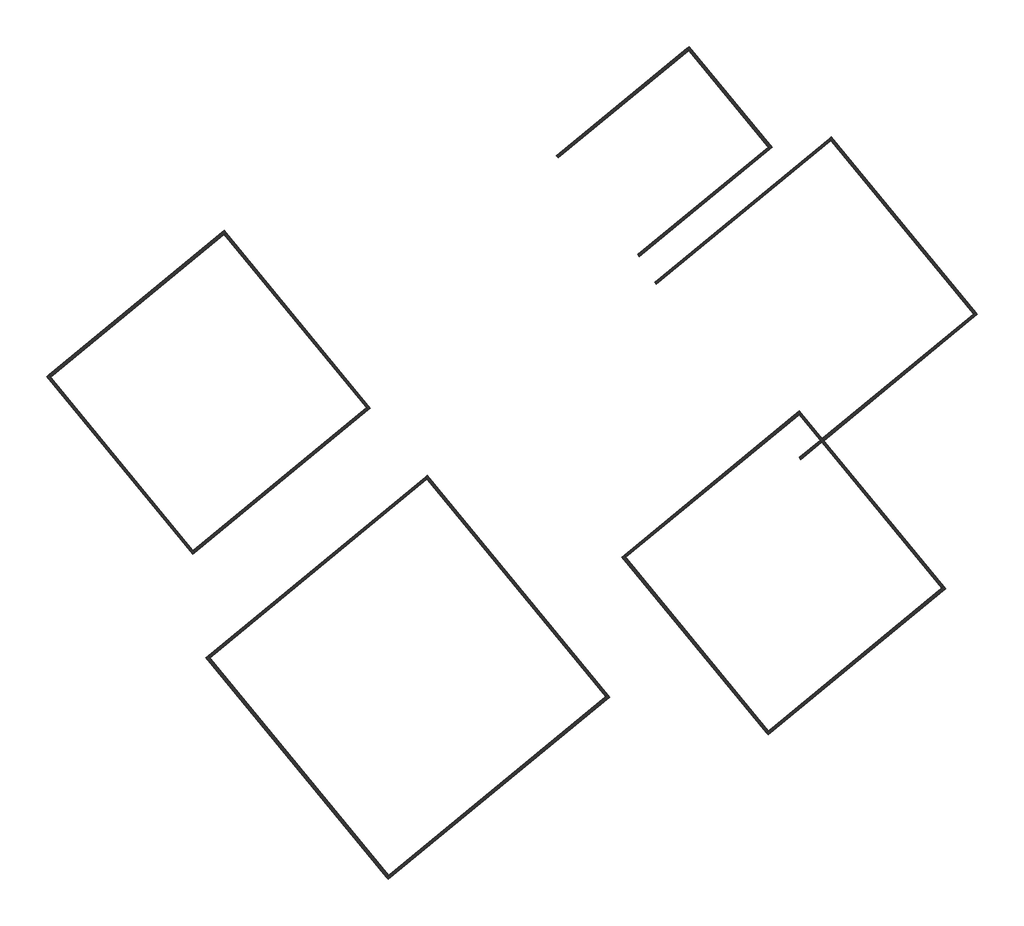
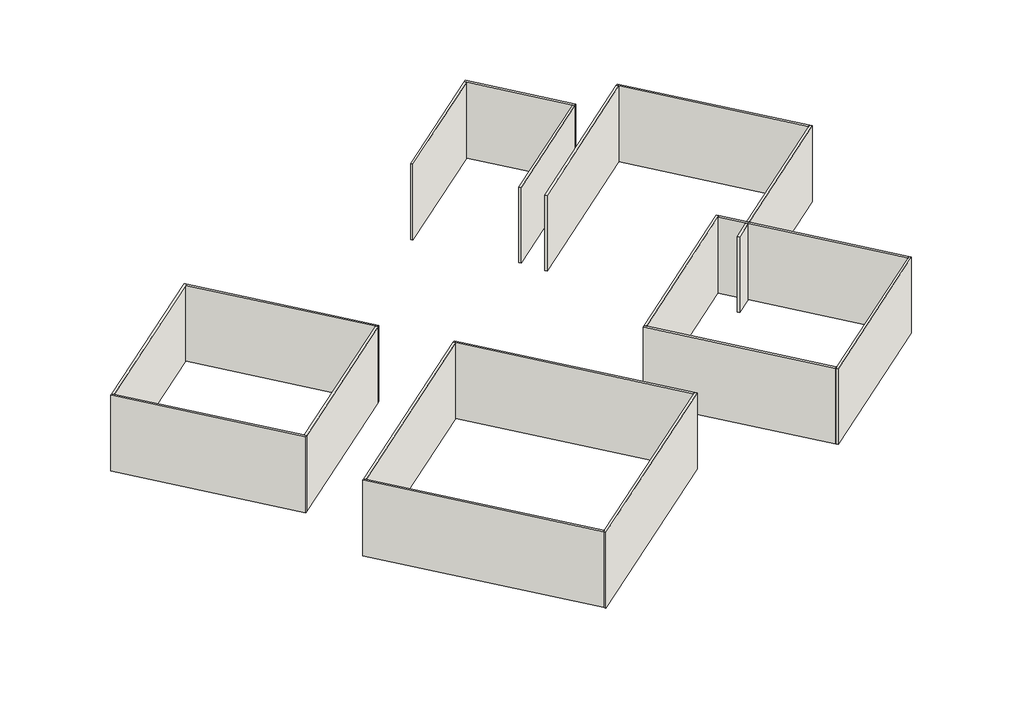
# One storey: 18 walls.
"""IFC4 building model written with IfcOpenShell, lengths in millimetres."""

from ifc_helpers import new_model, si_unit, frame, origin, place, context, project, spatial, polyline, outline, extrude, faceted_brep, element, save

model = new_model("IFC4")

# Units and contexts
model_context = context("Model", 3, world=origin())
ifc_project = project(units=[si_unit("LENGTHUNIT", "METRE", prefix="MILLI")], contexts=[model_context])

# Site, building, storey
site = spatial("IfcSite", under=ifc_project)
building = spatial("IfcBuilding", under=site)
storey = spatial("IfcBuildingStorey", under=building, Name="f3-展厅", Elevation=17500.0)

# Walls
placement = place(None, origin())
element("IfcWall", 1, ObjectType="aa-大理石-米黄色 - 200mm", at=placement, inside=storey, context=model_context, shape_type="Brep", body=[
    faceted_brep([(-29489.0476402, -25007.5608793, 17500.0), (-13891.5005151, -12171.8091024, 17500.0), (-13891.5005151, -12171.8091024, 24700.0), (-29489.0476402, -25007.5608793, 24700.0), (-29616.1342915, -24853.1297197, 17500.0), (-29616.1342915, -24853.1297197, 24700.0), (-29461.7031318, -24726.0430684, 24700.0), (-14173.018326, -12144.464594, 24700.0), (-14018.5871664, -12017.3779427, 24700.0), (-14018.5871664, -12017.3779427, 17500.0), (-14173.018326, -12144.464594, 17500.0), (-29461.7031318, -24726.0430684, 17500.0)], [[[0, 1, 2, 3]], [[4, 5, 6, 7, 8, 9, 10, 11]], [[1, 0, 4, 11, 10, 9]], [[3, 2, 8, 7, 6, 5]], [[2, 1, 9, 8]], [[0, 3, 5, 4]]]),
])
element("IfcWall", 2, ObjectType="aa-大理石-米黄色 - 200mm", at=placement, inside=storey, context=model_context, shape_type="Brep", body=[
    faceted_brep([(-14018.5871664, -12017.3779427, 17500.0), (-26727.2522921, 3425.7380228, 17500.0), (-26727.2522921, 3425.7380228, 24700.0), (-14018.5871664, -12017.3779427, 24700.0), (-14173.018326, -12144.464594, 17500.0), (-14173.018326, -12144.464594, 24700.0), (-26754.5968005, 3144.2202119, 24700.0), (-26881.6834517, 3298.6513715, 24700.0), (-26881.6834517, 3298.6513715, 17500.0), (-26754.5968005, 3144.2202119, 17500.0)], [[[0, 1, 2, 3]], [[4, 5, 6, 7, 8, 9]], [[1, 0, 4, 9, 8]], [[3, 2, 7, 6, 5]], [[0, 3, 5, 4]], [[2, 1, 8, 7]]]),
])
element("IfcWall", 3, ObjectType="aa-大理石-米黄色 - 200mm", at=placement, inside=storey, context=model_context, shape_type="Brep", body=[
    faceted_brep([(-42324.7994172, -9410.0137542, 17500.0), (-29616.1342915, -24853.1297197, 17500.0), (-29616.1342915, -24853.1297197, 24700.0), (-42324.7994172, -9410.0137542, 24700.0), (-42170.3682575, -9282.9271029, 17500.0), (-42170.3682575, -9282.9271029, 24700.0), (-42043.2816063, -9437.3582626, 24700.0), (-29461.7031318, -24726.0430684, 24700.0), (-29461.7031318, -24726.0430684, 17500.0), (-42043.2816063, -9437.3582626, 17500.0)], [[[0, 1, 2, 3]], [[4, 5, 6, 7, 8, 9]], [[1, 0, 4, 9, 8]], [[3, 2, 7, 6, 5]], [[2, 1, 8, 7]], [[0, 3, 5, 4]]]),
])
element("IfcWall", 4, ObjectType="aa-大理石-米黄色 - 200mm", at=placement, inside=storey, context=model_context, shape_type="SweptSolid", body=[
    extrude(outline(polyline([(-42170.3682575, -9282.9271029), (-26881.6834517, 3298.6513715), (-26754.5968005, 3144.2202119), (-42043.2816063, -9437.3582626), (-42170.3682575, -9282.9271029)])), frame((0.0, 0.0, 17500.0), z_axis=(0.0, 0.0, 1.0), x_axis=(1.0, 0.0, 0.0)), (0.0, 0.0, 1.0), 7200.0),
])
element("IfcWall", 5, ObjectType="aa-大理石-米黄色 - 200mm", at=placement, inside=storey, context=model_context, shape_type="Brep", body=[
    faceted_brep([(-53539.2738644, 10380.4187427, 17500.0), (-43245.2551126, -2128.5051893, 17500.0), (-43245.2551126, -2128.5051893, 24700.0), (-53539.2738644, 10380.4187427, 24700.0), (-53384.8427048, 10507.505394, 17500.0), (-53384.8427048, 10507.505394, 24700.0), (-53257.7560535, 10353.0742343, 24700.0), (-43217.9106042, -1846.9873784, 24700.0), (-43090.823953, -2001.418538, 24700.0), (-43090.823953, -2001.418538, 17500.0), (-43217.9106042, -1846.9873784, 17500.0), (-53257.7560535, 10353.0742343, 17500.0)], [[[0, 1, 2, 3]], [[4, 5, 6, 7, 8, 9, 10, 11]], [[1, 0, 4, 11, 10, 9]], [[3, 2, 8, 7, 6, 5]], [[0, 3, 5, 4]], [[2, 1, 9, 8]]]),
])
element("IfcWall", 6, ObjectType="aa-大理石-米黄色 - 200mm", at=placement, inside=storey, context=model_context, shape_type="Brep", body=[
    faceted_brep([(-41030.3499324, 20674.4374946, 17500.0), (-53384.8427048, 10507.505394, 17500.0), (-53384.8427048, 10507.505394, 24700.0), (-41030.3499324, 20674.4374946, 24700.0), (-40903.2632812, 20520.0063349, 17500.0), (-40903.2632812, 20520.0063349, 24700.0), (-41057.6944408, 20392.9196836, 24700.0), (-53257.7560535, 10353.0742343, 24700.0), (-53257.7560535, 10353.0742343, 17500.0), (-41057.6944408, 20392.9196836, 17500.0)], [[[0, 1, 2, 3]], [[4, 5, 6, 7, 8, 9]], [[1, 0, 4, 9, 8]], [[3, 2, 7, 6, 5]], [[2, 1, 8, 7]], [[0, 3, 5, 4]]]),
])
element("IfcWall", 7, ObjectType="aa-大理石-米黄色 - 200mm", at=placement, inside=storey, context=model_context, shape_type="Brep", body=[
    faceted_brep([(-30736.3311806, 8165.5135625, 17500.0), (-40903.2632812, 20520.0063349, 17500.0), (-40903.2632812, 20520.0063349, 24700.0), (-30736.3311806, 8165.5135625, 24700.0), (-30890.7623403, 8038.4269113, 17500.0), (-30890.7623403, 8038.4269113, 24700.0), (-31017.8489915, 8192.8580709, 24700.0), (-41057.6944408, 20392.9196836, 24700.0), (-41057.6944408, 20392.9196836, 17500.0), (-31017.8489915, 8192.8580709, 17500.0)], [[[0, 1, 2, 3]], [[4, 5, 6, 7, 8, 9]], [[1, 0, 4, 9, 8]], [[3, 2, 7, 6, 5]], [[2, 1, 8, 7]], [[0, 3, 5, 4]]]),
])
element("IfcWall", 8, ObjectType="aa-大理石-米黄色 - 200mm", at=placement, inside=storey, context=model_context, shape_type="SweptSolid", body=[
    extrude(outline(polyline([(-30890.7623403, 8038.4269113), (-43090.823953, -2001.418538), (-43217.9106042, -1846.9873784), (-31017.8489915, 8192.8580709), (-30890.7623403, 8038.4269113)])), frame((0.0, 0.0, 17500.0), z_axis=(0.0, 0.0, 1.0), x_axis=(1.0, 0.0, 0.0)), (0.0, 0.0, 1.0), 7200.0),
])
element("IfcWall", 9, ObjectType="aa-大理石-米黄色 - 200mm", at=placement, inside=storey, context=model_context, shape_type="Brep", body=[
    faceted_brep([(-2742.3908548, -14827.0816231, 17500.0), (9766.5330772, -4533.0628713, 17500.0), (9766.5330772, -4533.0628713, 24700.0), (-2742.3908548, -14827.0816231, 24700.0), (-2869.4775061, -14672.6504634, 17500.0), (-2869.4775061, -14672.6504634, 24700.0), (-2715.0463464, -14545.5638122, 24700.0), (9485.0152663, -4505.7183629, 24700.0), (9639.446426, -4378.6317116, 24700.0), (9639.446426, -4378.6317116, 17500.0), (9485.0152663, -4505.7183629, 17500.0), (-2715.0463464, -14545.5638122, 17500.0)], [[[0, 1, 2, 3]], [[4, 5, 6, 7, 8, 9, 10, 11]], [[1, 0, 4, 11, 10, 9]], [[3, 2, 8, 7, 6, 5]], [[0, 3, 5, 4]], [[2, 1, 9, 8]]]),
])
element("IfcWall", 10, ObjectType="aa-大理石-米黄色 - 200mm", at=placement, inside=storey, context=model_context, shape_type="Brep", body=[
    faceted_brep([(-13036.4096066, -2318.157691, 17500.0), (-2869.4775061, -14672.6504634, 17500.0), (-2869.4775061, -14672.6504634, 24700.0), (-13036.4096066, -2318.157691, 24700.0), (-12881.978447, -2191.0710398, 17500.0), (-12881.978447, -2191.0710398, 24700.0), (-12754.8917957, -2345.5021994, 24700.0), (-2715.0463464, -14545.5638122, 24700.0), (-2715.0463464, -14545.5638122, 17500.0), (-12754.8917957, -2345.5021994, 17500.0)], [[[0, 1, 2, 3]], [[4, 5, 6, 7, 8, 9]], [[1, 0, 4, 9, 8]], [[3, 2, 7, 6, 5]], [[2, 1, 8, 7]], [[0, 3, 5, 4]]]),
])
element("IfcWall", 11, ObjectType="aa-大理石-米黄色 - 200mm", at=placement, inside=storey, context=model_context, shape_type="Brep", body=[
    faceted_brep([(-527.4856746, 7975.8610608, 17500.0), (-12881.978447, -2191.0710398, 17500.0), (-12881.978447, -2191.0710398, 24700.0), (-527.4856746, 7975.8610608, 24700.0), (-400.3990233, 7821.4299011, 17500.0), (-400.3990233, 7821.4299011, 24700.0), (-554.830183, 7694.3432499, 24700.0), (-12754.8917957, -2345.5021994, 24700.0), (-12754.8917957, -2345.5021994, 17500.0), (-554.830183, 7694.3432499, 17500.0)], [[[0, 1, 2, 3]], [[4, 5, 6, 7, 8, 9]], [[1, 0, 4, 9, 8]], [[3, 2, 7, 6, 5]], [[2, 1, 8, 7]], [[0, 3, 5, 4]]]),
])
element("IfcWall", 12, ObjectType="aa-大理石-米黄色 - 200mm", at=placement, inside=storey, context=model_context, shape_type="Brep", body=[
    faceted_brep([(9639.446426, -4378.6317116, 17500.0), (1199.9237396, 5876.7748358, 17500.0), (1072.8370883, 6031.2059954, 17500.0), (-400.3990233, 7821.4299011, 17500.0), (-400.3990233, 7821.4299011, 24700.0), (1072.8370883, 6031.2059954, 24700.0), (1199.9237396, 5876.7748358, 24700.0), (9639.446426, -4378.6317116, 24700.0), (9485.0152663, -4505.7183629, 17500.0), (9485.0152663, -4505.7183629, 24700.0), (1045.4925799, 5749.6881845, 24700.0), (918.4059287, 5904.1193442, 24700.0), (-554.830183, 7694.3432499, 24700.0), (-554.830183, 7694.3432499, 17500.0), (918.4059287, 5904.1193442, 17500.0), (1045.4925799, 5749.6881845, 17500.0)], [[[0, 1, 2, 3, 4, 5, 6, 7]], [[8, 9, 10, 11, 12, 13, 14, 15]], [[3, 2, 1, 0, 8, 15, 14, 13]], [[7, 6, 5, 4, 12, 11, 10, 9]], [[0, 7, 9, 8]], [[4, 3, 13, 12]]]),
])
element("IfcWall", 13, ObjectType="aa-大理石-米黄色 - 200mm", at=placement, inside=storey, context=model_context, shape_type="Brep", body=[
    faceted_brep([(-429.0438457, 4536.2420322, 24700.0), (-429.0438457, 4536.2420322, 17500.0), (1045.4925799, 5749.6881845, 17500.0), (1045.4925799, 5749.6881845, 24700.0), (-556.1304969, 4690.6731918, 17500.0), (-556.1304969, 4690.6731918, 24700.0), (918.4059287, 5904.1193442, 24700.0), (918.4059287, 5904.1193442, 17500.0)], [[[0, 1, 2, 3]], [[4, 5, 6, 7]], [[1, 4, 7, 2]], [[5, 0, 3, 6]], [[1, 0, 5, 4]], [[3, 2, 7, 6]]]),
    faceted_brep([(12002.6645065, 14766.7174583, 17500.0), (12002.6645065, 14766.7174583, 24700.0), (1199.9237396, 5876.7748358, 24700.0), (1199.9237396, 5876.7748358, 17500.0), (11875.5778553, 14921.148618, 24700.0), (11875.5778553, 14921.148618, 17500.0), (11721.1466956, 14794.0619667, 17500.0), (1072.8370883, 6031.2059954, 17500.0), (1072.8370883, 6031.2059954, 24700.0), (11721.1466956, 14794.0619667, 24700.0)], [[[0, 1, 2, 3]], [[4, 5, 6, 7, 8, 9]], [[5, 0, 3, 7, 6]], [[1, 4, 9, 8, 2]], [[3, 2, 8, 7]], [[1, 0, 5, 4]]]),
])
element("IfcWall", 14, ObjectType="aa-大理石-米黄色 - 200mm", at=placement, inside=storey, context=model_context, shape_type="Brep", body=[
    faceted_brep([(11875.5778553, 14921.148618, 17500.0), (1708.6457547, 27275.6413904, 17500.0), (1708.6457547, 27275.6413904, 24700.0), (11875.5778553, 14921.148618, 24700.0), (11721.1466956, 14794.0619667, 17500.0), (11721.1466956, 14794.0619667, 24700.0), (1681.3012463, 26994.1235795, 24700.0), (1554.2145951, 27148.5547391, 24700.0), (1554.2145951, 27148.5547391, 17500.0), (1681.3012463, 26994.1235795, 17500.0)], [[[0, 1, 2, 3]], [[4, 5, 6, 7, 8, 9]], [[1, 0, 4, 9, 8]], [[3, 2, 7, 6, 5]], [[0, 3, 5, 4]], [[2, 1, 8, 7]]]),
])
element("IfcWall", 15, ObjectType="aa-大理石-米黄色 - 200mm", at=placement, inside=storey, context=model_context, shape_type="SweptSolid", body=[
    extrude(outline(polyline([(-10723.0625975, 17045.1659642), (1554.2145951, 27148.5547391), (1681.3012463, 26994.1235795), (-10595.9759462, 16890.7348045), (-10723.0625975, 17045.1659642)])), frame((0.0, 0.0, 17500.0), z_axis=(0.0, 0.0, 1.0), x_axis=(1.0, 0.0, 0.0)), (0.0, 0.0, 1.0), 7200.0),
])
element("IfcWall", 16, ObjectType="aa-大理石-米黄色 - 200mm", at=placement, inside=storey, context=model_context, shape_type="Brep", body=[
    faceted_brep([(-2450.3096158, 26520.6035137, 17500.0), (-8296.2955736, 33624.4368578, 17500.0), (-8296.2955736, 33624.4368578, 24700.0), (-2450.3096158, 26520.6035137, 24700.0), (-2604.7407754, 26393.5168624, 17500.0), (-2604.7407754, 26393.5168624, 24700.0), (-2731.8274267, 26547.9480221, 24700.0), (-8323.640082, 33342.9190469, 24700.0), (-8450.7267332, 33497.3502065, 24700.0), (-8450.7267332, 33497.3502065, 17500.0), (-8323.640082, 33342.9190469, 17500.0), (-2731.8274267, 26547.9480221, 17500.0)], [[[0, 1, 2, 3]], [[4, 5, 6, 7, 8, 9, 10, 11]], [[1, 0, 4, 11, 10, 9]], [[3, 2, 8, 7, 6, 5]], [[0, 3, 5, 4]], [[2, 1, 9, 8]]]),
])
element("IfcWall", 17, ObjectType="aa-大理石-米黄色 - 200mm", at=placement, inside=storey, context=model_context, shape_type="SweptSolid", body=[
    extrude(outline(polyline([(-2604.7407754, 26393.5168624), (-11793.3947749, 18831.8611126), (-11920.4814261, 18986.2922723), (-2731.8274267, 26547.9480221), (-2604.7407754, 26393.5168624)])), frame((0.0, 0.0, 17500.0), z_axis=(0.0, 0.0, 1.0), x_axis=(1.0, 0.0, 0.0)), (0.0, 0.0, 1.0), 7200.0),
])
element("IfcWall", 18, ObjectType="aa-大理石-米黄色 - 200mm", at=placement, inside=storey, context=model_context, shape_type="SweptSolid", body=[
    extrude(outline(polyline([(-17639.3807327, 25935.6944567), (-8450.7267332, 33497.3502065), (-8323.640082, 33342.9190469), (-17512.2940814, 25781.2632971), (-17639.3807327, 25935.6944567)])), frame((0.0, 0.0, 17500.0), z_axis=(0.0, 0.0, 1.0), x_axis=(1.0, 0.0, 0.0)), (0.0, 0.0, 1.0), 7200.0),
])

save(model, "model.ifc")

# Revit data of these elements
# Type "aa-大理石-米黄色 - 200mm"
#   Width = 200 mm
#   Layers, outside or top first: 200 mm "aa-大理石-米黄色" (function 1)
# Elements 1, 2, 3, 4, 5, 6, 7, 8, 9, 10, 11, 12, 13, 14, 15, 16, 17, 18 (IfcWall, "aa-大理石-米黄色 - 200mm")
#   Top Offset = 0 mm
#   Base Offset = 0 mm
#   wall height = 7200 mm
#   Phase Created = 新构造
#   Base Constraint = f3-展厅
#   Top Constraint = 屋顶
#   Materials on its faces: "aa-大理石-米黄色"
# Materials
#   "aa-大理石-米黄色": class "石材", colour RGB 127 127 127, transparency 0, Cost = 0
